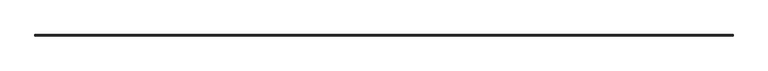
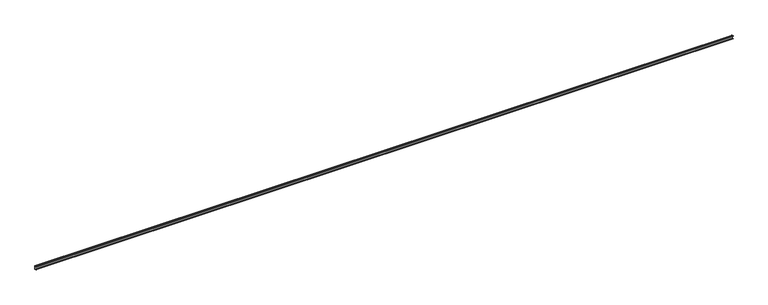
"""IFC4 building model written with IfcOpenShell, lengths in millimetres: beam geometry, 0912_Steel Framing_LC_KDS3530 : H_SB_AR_B03_LC-200x75x25x3.2."""

from ifc_helpers import new_model, si_unit, point, frame, frame_2d, origin, place, context, project, spatial, polyline, circle_curve, trimmed, segment, composite_curve, outline, extrude, source, transform, mapped, element, save


def beam_1c6e9d3a(model_context):
    return source(origin(), model_context, "Body", "SweptSolid", [
        extrude(outline(composite_curve([segment(polyline([(18.6, 87.5), (18.6, -87.5)]), True, "CONTINUOUS"), segment(trimmed(circle_curve(frame_2d((6.1, -87.5)), 12.5), [point((18.6, -87.5))], [point((6.1, -100.0))], False, "CARTESIAN"), True, "CONTINUOUS"), segment(polyline([(6.1, -100.0), (-43.9, -100.0)]), True, "CONTINUOUS"), segment(trimmed(circle_curve(frame_2d((-43.9, -87.5)), 12.5), [point((-43.9, -100.0))], [point((-56.4, -87.5))], False, "CARTESIAN"), True, "CONTINUOUS"), segment(polyline([(-56.4, -87.5), (-56.4, -75.0), (-51.9, -75.0), (-51.9, -87.5)]), True, "CONTINUOUS"), segment(trimmed(circle_curve(frame_2d((-43.9, -87.5)), 8.0), [point((-51.9, -87.5))], [point((-43.9, -95.5))], True, "CARTESIAN"), True, "CONTINUOUS"), segment(polyline([(-43.9, -95.5), (6.1, -95.5)]), True, "CONTINUOUS"), segment(trimmed(circle_curve(frame_2d((6.1, -87.5)), 8.0), [point((6.1, -95.5))], [point((14.1, -87.5))], True, "CARTESIAN"), True, "CONTINUOUS"), segment(polyline([(14.1, -87.5), (14.1, 87.5)]), True, "CONTINUOUS"), segment(trimmed(circle_curve(frame_2d((6.1, 87.5)), 8.0), [point((14.1, 87.5))], [point((6.1, 95.5))], True, "CARTESIAN"), True, "CONTINUOUS"), segment(polyline([(6.1, 95.5), (-41.1, 95.5)]), True, "CONTINUOUS"), segment(trimmed(circle_curve(frame_2d((-41.1, 87.5)), 8.0), [point((-41.1, 95.5))], [point((-49.1, 87.5))], True, "CARTESIAN"), True, "CONTINUOUS"), segment(polyline([(-49.1, 87.5), (-49.1, 75.0), (-53.6, 75.0), (-53.6, 87.5)]), True, "CONTINUOUS"), segment(trimmed(circle_curve(frame_2d((-41.1, 87.5)), 12.5), [point((-53.6, 87.5))], [point((-41.1, 100.0))], False, "CARTESIAN"), True, "CONTINUOUS"), segment(polyline([(-41.1, 100.0), (6.1, 100.0)]), True, "CONTINUOUS"), segment(trimmed(circle_curve(frame_2d((6.1, 87.5)), 12.5), [point((6.1, 100.0))], [point((18.6, 87.5))], False, "CARTESIAN"), True, "CONTINUOUS")], self_intersect=False)), frame((-19660.0, 0.0, 0.0), z_axis=(1.0, 0.0, 0.0), x_axis=(0.0, 1.0, 0.0)), (0.0, 0.0, 1.0), 39299.0),
    ])


if __name__ == "__main__":
    model = new_model("IFC4")
    model_context = context("Model", 3, world=origin())
    ifc_project = project(units=[si_unit("LENGTHUNIT", "METRE", prefix="MILLI")], contexts=[model_context])
    site = spatial("IfcSite", under=ifc_project)
    building = spatial("IfcBuilding", under=site)
    placement = place(None, origin())
    beam_shape = beam_1c6e9d3a(model_context)
    element("IfcBeam", 1, ObjectType="0912_Steel Framing_LC_KDS3530 : H_SB_AR_B03_LC-200x75x25x3.2", at=placement, inside=building, context=model_context, shape_type="MappedRepresentation", body=[
        mapped(beam_shape, transform((0.0, 0.0, 0.0), x_axis=(1.0, 0.0, 0.0), y_axis=(0.0, 1.0, 0.0), z_axis=(0.0, 0.0, 1.0))),
    ])
    save(model, "model.ifc")

# Revit data of these elements
# Type "0912_Steel Framing_LC_KDS3530 : H_SB_AR_B03_LC-200x75x25x3.2"
#   r = 8 mm
#   d = 25 mm
#   R = 11.2 mm
#   Perimeter = 0.78 m²/m
#   Nominal Weight = 14.00 kgf/m
#   Length [instance default] = 1000 mm
#   B = 75 mm
#   H = 200 mm
#   tw = 3.2 mm
#   x = 18.6 mm
#   A = 1.00 m²
#   Structural Material [instance default] = Steel, 45-345
#   Assembly Code = ""
# Element 1 (IfcBeam, "0912_Steel Framing_LC_KDS3530 : H_SB_AR_B03_LC-200x75x25x3.2")
#   Structural Material = Steel ASTM A36
#   Materials on its faces: "Steel ASTM A36"
# Materials
#   "Steel, 45-345": class "Metal", colour RGB 189 187 185, transparency 0, Description = "Steel 345 MPa", Cost = 0
#   "Steel ASTM A36": class "Metal", colour RGB 199 199 199, transparency 0, Description = "Structural steel, ASTM A36 Grade B, mill finish", Cost = 0
